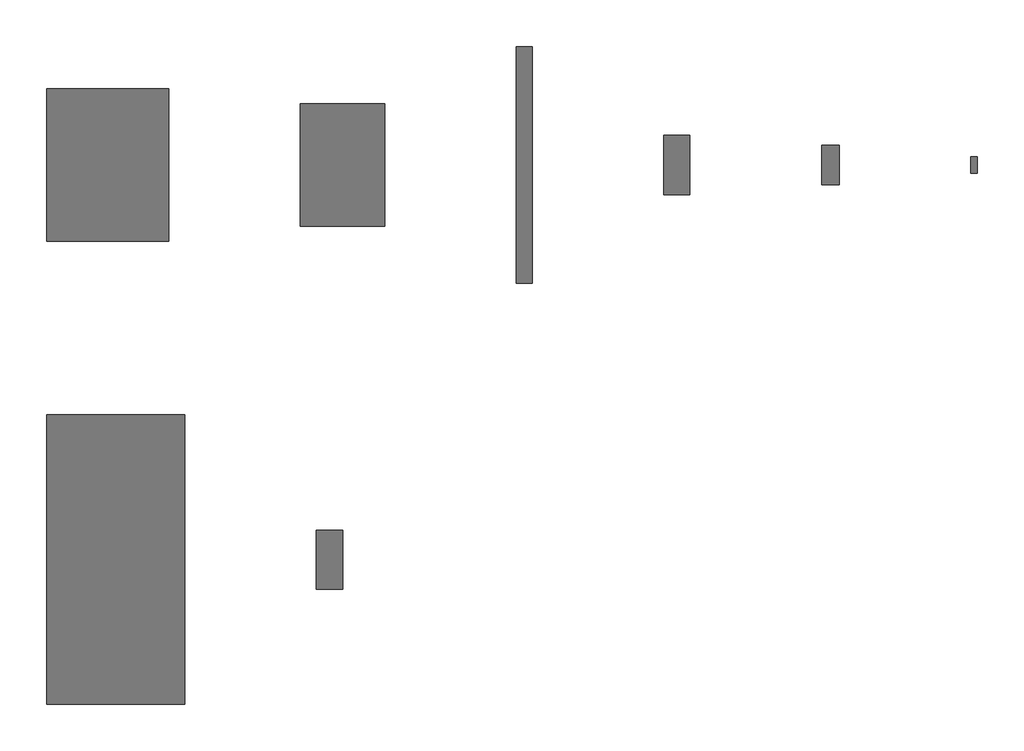
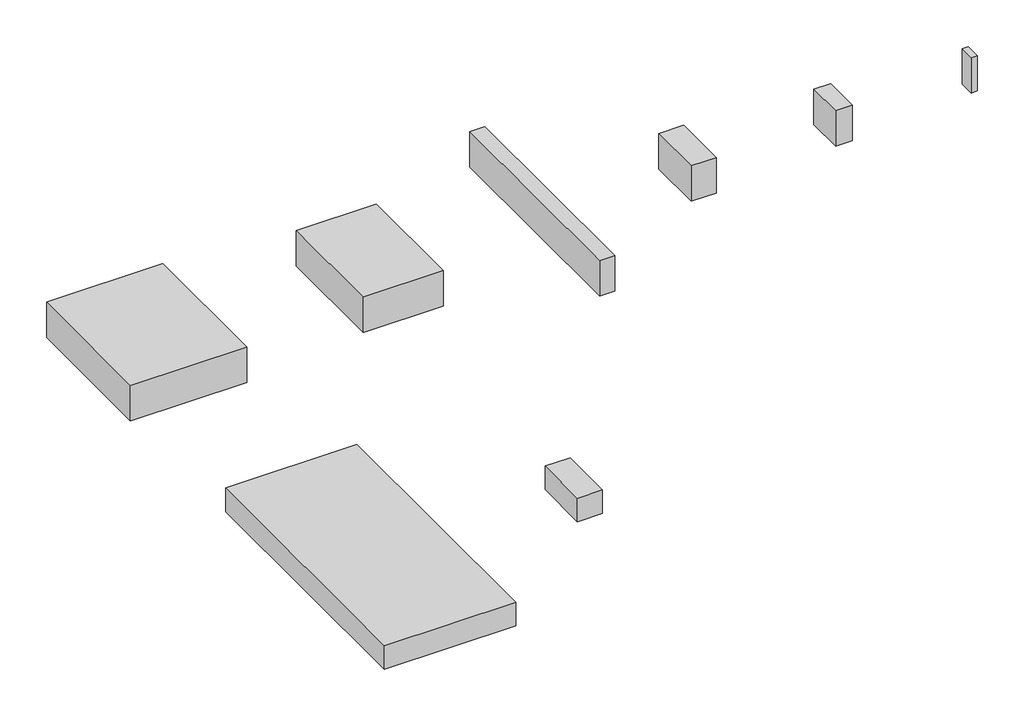
# One storey: 8 proxies.
"""IFC4 building model written with IfcOpenShell, lengths in millimetres."""

import ifcopenshell
import ifcopenshell.guid

model = None  # the IFC model being written
_history = None  # IfcOwnerHistory: only IFC2X3 demands one
_inside = {}  # id of a spatial element -> (the spatial element, [elements in it])
_under = {}  # id of a project, library or spatial element -> (it, [spatial elements below it])
_declared = {}  # id of a project -> (the project, [libraries it declares])
_typed = {}  # id of a type object -> (the type object, [elements of that type])
_made_of = {}  # id of a material, layer set ... -> (it, [elements and type objects made of it])


def new_model(schema):
    """Start an empty IFC model of exactly this schema.

    Asked for "IFC4X3", IfcOpenShell would pick the latest addendum, in which some entities
    have other attributes; the version numbers below select the first issue.
    IFC2X3 requires an IfcOwnerHistory on every rooted entity: one is made here for all.
    """
    global model, _history
    if schema == "IFC4X3":
        model = ifcopenshell.file(schema_version=(4, 3, 0, 0))
    else:
        model = ifcopenshell.file(schema=schema)
    _inside.clear()
    _under.clear()
    _declared.clear()
    _typed.clear()
    _made_of.clear()
    _history = None
    if model.schema == "IFC2X3":
        org = make("IfcOrganization", Name="unknown")
        user = make(
            "IfcPersonAndOrganization",
            ThePerson=make("IfcPerson", FamilyName="unknown"),
            TheOrganization=org,
        )
        app = make(
            "IfcApplication",
            ApplicationDeveloper=org,
            Version="unknown",
            ApplicationFullName="unknown",
            ApplicationIdentifier="unknown",
        )
        _history = make(
            "IfcOwnerHistory",
            OwningUser=user,
            OwningApplication=app,
            ChangeAction="ADDED",
            CreationDate=0,
        )
    return model


def make(cls, **values):
    """One entity of the class cls with the attributes given. An attribute that is None is left unset."""
    return model.create_entity(
        cls, **{name: value for name, value in values.items() if value is not None}
    )


def rooted(cls, **values):
    """An entity with a GlobalId (a new one), such as an element, a storey or a relation."""
    return make(cls, GlobalId=ifcopenshell.guid.new(), OwnerHistory=_history, **values)


def si_unit(unit_type, name, prefix=None):
    """IfcSIUnit, for example si_unit("LENGTHUNIT", "METRE", prefix="MILLI")."""
    return make("IfcSIUnit", UnitType=unit_type, Prefix=prefix, Name=name)


def assignment(units):
    """IfcUnitAssignment: the units of a project."""
    return None if units is None else make("IfcUnitAssignment", Units=units)


def point(xyz):
    """IfcCartesianPoint."""
    return None if xyz is None else make("IfcCartesianPoint", Coordinates=xyz)


def direction(xyz):
    """IfcDirection."""
    return None if xyz is None else make("IfcDirection", DirectionRatios=xyz)


def frame(location, z_axis=None, x_axis=None):
    """IfcAxis2Placement3D, a coordinate frame: its origin and axes. An axis left out is left unset."""
    return make(
        "IfcAxis2Placement3D",
        Location=point(location),
        Axis=direction(z_axis),
        RefDirection=direction(x_axis),
    )


def origin():
    """The frame at (0, 0, 0) with its axes left unset."""
    return frame((0.0, 0.0, 0.0))


def origin_with_axes():
    """The frame at (0, 0, 0) with the z axis (0, 0, 1) and the x axis (1, 0, 0) written out."""
    return frame((0.0, 0.0, 0.0), z_axis=(0.0, 0.0, 1.0), x_axis=(1.0, 0.0, 0.0))


def place(relative_to, where):
    """IfcLocalPlacement: puts the frame where relative to a parent placement (None: the world)."""
    return make(
        "IfcLocalPlacement", PlacementRelTo=relative_to, RelativePlacement=where
    )


def context(
    kind, dimensions, precision=None, world=None, true_north=None, identifier=None
):
    """IfcGeometricRepresentationContext, for example the 3D "Model" context."""
    return make(
        "IfcGeometricRepresentationContext",
        ContextIdentifier=identifier,
        ContextType=kind,
        CoordinateSpaceDimension=dimensions,
        Precision=precision,
        WorldCoordinateSystem=world,
        TrueNorth=true_north,
    )


def project(units=None, contexts=None):
    """IfcProject with its units and contexts."""
    return rooted(
        "IfcProject",
        Name="project",
        RepresentationContexts=contexts,
        UnitsInContext=assignment(units),
    )


def spatial(cls, under=None, at=None, **own):
    """A site, building, storey or space (cls), placed at a placement, below another one or the project."""
    s = rooted(cls, ObjectPlacement=at, **own)
    if under is not None:
        _under.setdefault(under.id(), (under, []))[1].append(s)
    return s


def polyline(points):
    """IfcPolyline through the points."""
    return make("IfcPolyline", Points=[point(p) for p in points])


def outline(outer, holes=None, kind="AREA"):
    """IfcArbitraryClosedProfileDef: a profile drawn as a closed curve; with holes, ...WithVoids."""
    if holes is None:
        return make("IfcArbitraryClosedProfileDef", ProfileType=kind, OuterCurve=outer)
    return make(
        "IfcArbitraryProfileDefWithVoids",
        ProfileType=kind,
        OuterCurve=outer,
        InnerCurves=holes,
    )


def extrude(swept, where, along, depth):
    """IfcExtrudedAreaSolid: the profile swept, set in the frame where, extruded along a direction by depth."""
    return make(
        "IfcExtrudedAreaSolid",
        SweptArea=swept,
        Position=where,
        ExtrudedDirection=direction(along),
        Depth=depth,
    )


def shape(context_of_items, identifier, shape_type, items):
    """IfcShapeRepresentation: the items that make up one representation, for example the "Body"."""
    return make(
        "IfcShapeRepresentation",
        ContextOfItems=context_of_items,
        RepresentationIdentifier=identifier,
        RepresentationType=shape_type,
        Items=items,
    )


def source(mapping_origin, context_of_items, identifier, shape_type, items):
    """IfcRepresentationMap: a shape defined once, which mapped items show again and again."""
    return make(
        "IfcRepresentationMap",
        MappingOrigin=mapping_origin,
        MappedRepresentation=shape(context_of_items, identifier, shape_type, items),
    )


def transform(
    local_origin,
    x_axis=None,
    y_axis=None,
    z_axis=None,
    scale=None,
    scale2=None,
    scale3=None,
    uniform=True,
):
    """IfcCartesianTransformationOperator3D, or its non-uniform kind. x_axis, y_axis, z_axis: its Axis1, 2, 3."""
    if uniform:
        return make(
            "IfcCartesianTransformationOperator3D",
            Axis1=direction(x_axis),
            Axis2=direction(y_axis),
            LocalOrigin=point(local_origin),
            Scale=scale,
            Axis3=direction(z_axis),
        )
    return make(
        "IfcCartesianTransformationOperator3DnonUniform",
        Axis1=direction(x_axis),
        Axis2=direction(y_axis),
        LocalOrigin=point(local_origin),
        Scale=scale,
        Axis3=direction(z_axis),
        Scale2=scale2,
        Scale3=scale3,
    )


def mapped(mapping_source, mapping_target):
    """IfcMappedItem: shows the shape of a source again, moved by a transform."""
    return make(
        "IfcMappedItem", MappingSource=mapping_source, MappingTarget=mapping_target
    )


def made_of(thing, what):
    """Note that an element or type object is made of a material, layer set ...; save() writes the relation."""
    if what is not None:
        _made_of.setdefault(what.id(), (what, []))[1].append(thing)
    return thing


def element(
    cls,
    number,
    at=None,
    inside=None,
    cuts=None,
    type_object=None,
    material=None,
    context=None,
    identifier="Body",
    shape_type=None,
    held_by="IfcProductDefinitionShape",
    body=None,
    shapes=None,
    **own,
):
    """One element of the class cls, such as IfcWall. Its Tag is "e" and its number.

    at: its placement. inside: the storey or other place that contains it. cuts: it is an
    opening in that element (IfcRelVoidsElement). A single representation is given by context,
    identifier, shape_type and body (its items); several are given by shapes. held_by: the class
    of the entity that holds the representations. save() writes the other relations.
    """
    e = rooted(cls, Tag="e%d" % number, ObjectPlacement=at, **own)
    if body is not None:
        shapes = [shape(context, identifier, shape_type, body)]
    if shapes is not None:
        e.Representation = make(held_by, Representations=shapes)
    if inside is not None:
        _inside.setdefault(inside.id(), (inside, []))[1].append(e)
    if cuts is not None:
        rooted(
            "IfcRelVoidsElement", RelatingBuildingElement=cuts, RelatedOpeningElement=e
        )
    if type_object is not None:
        _typed.setdefault(type_object.id(), (type_object, []))[1].append(e)
    return made_of(e, material)


def aggregate(whole, parts):
    """IfcRelAggregates: a whole, such as a stair, and the parts it consists of."""
    return rooted("IfcRelAggregates", RelatingObject=whole, RelatedObjects=parts)


def save(model, path):
    """Write the relations noted so far, then the file.

    IfcRelAggregates (storeys below a building ...), IfcRelContainedInSpatialStructure (elements
    in a storey), IfcRelDefinesByType, IfcRelAssociatesMaterial and IfcRelDeclares: one each for
    every whole, place, type object, material and project.
    """
    for whole, parts in _under.values():
        aggregate(whole, parts)
    for where, things in _inside.values():
        rooted(
            "IfcRelContainedInSpatialStructure",
            RelatedElements=things,
            RelatingStructure=where,
        )
    for kind, things in _typed.values():
        rooted("IfcRelDefinesByType", RelatedObjects=things, RelatingType=kind)
    for what, things in _made_of.values():
        rooted("IfcRelAssociatesMaterial", RelatedObjects=things, RelatingMaterial=what)
    for by, libraries in _declared.values():
        rooted("IfcRelDeclares", RelatingContext=by, RelatedDefinitions=libraries)
    model.write(path)


def generic_models_29bcd6f9(model_context):
    return source(origin(), model_context, "Body", "SweptSolid", [
        extrude(outline(polyline([(2000.0, 4500.0), (2000.0, -4500.0), (-2000.0, -4500.0), (-2000.0, 4500.0), (2000.0, 4500.0)])), origin_with_axes(), (0.0, 0.0, 1.0), 6000.0),
    ])


def generic_models_a454a2aa(model_context):
    return source(origin(), model_context, "Body", "SweptSolid", [
        extrude(outline(polyline([(10500.0, 22000.0), (10500.0, -22000.0), (-10500.0, -22000.0), (-10500.0, 22000.0), (10500.0, 22000.0)])), origin_with_axes(), (0.0, 0.0, 1.0), 4000.0),
    ])


def generic_models_73802227(model_context):
    return source(origin(), model_context, "Body", "SweptSolid", [
        extrude(outline(polyline([(2000.0, 4500.0), (2000.0, -4500.0), (-2000.0, -4500.0), (-2000.0, 4500.0), (2000.0, 4500.0)])), origin_with_axes(), (0.0, 0.0, 1.0), 4000.0),
    ])


def generic_models_d82b1902(model_context):
    return source(origin(), model_context, "Body", "SweptSolid", [
        extrude(outline(polyline([(9300.0, 11600.0), (9300.0, -11600.0), (-9300.0, -11600.0), (-9300.0, 11600.0), (9300.0, 11600.0)])), origin_with_axes(), (0.0, 0.0, 1.0), 6000.0),
    ])


def generic_models_21711933(model_context):
    return source(origin(), model_context, "Body", "SweptSolid", [
        extrude(outline(polyline([(6400.0, 9300.0), (6400.0, -9300.0), (-6400.0, -9300.0), (-6400.0, 9300.0), (6400.0, 9300.0)])), origin_with_axes(), (0.0, 0.0, 1.0), 6000.0),
    ])


def generic_models_03d31222(model_context):
    return source(origin(), model_context, "Body", "SweptSolid", [
        extrude(outline(polyline([(1200.0, 18000.0), (1200.0, -18000.0), (-1200.0, -18000.0), (-1200.0, 18000.0), (1200.0, 18000.0)])), origin_with_axes(), (0.0, 0.0, 1.0), 6000.0),
    ])


def generic_models_5634f436(model_context):
    return source(origin(), model_context, "Body", "SweptSolid", [
        extrude(outline(polyline([(1350.0, 3000.0), (1350.0, -3000.0), (-1350.0, -3000.0), (-1350.0, 3000.0), (1350.0, 3000.0)])), origin_with_axes(), (0.0, 0.0, 1.0), 6000.0),
    ])


def generic_models_71e2440f(model_context):
    return source(origin(), model_context, "Body", "SweptSolid", [
        extrude(outline(polyline([(500.0, 1250.0), (500.0, -1250.0), (-500.0, -1250.0), (-500.0, 1250.0), (500.0, 1250.0)])), origin_with_axes(), (0.0, 0.0, 1.0), 6000.0),
    ])


model = new_model("IFC4")

# Units and contexts
model_context = context("Model", 3, world=origin())
ifc_project = project(units=[si_unit("LENGTHUNIT", "METRE", prefix="MILLI")], contexts=[model_context])

# Site, building, storey
site = spatial("IfcSite", under=ifc_project)
building = spatial("IfcBuilding", under=site)
storey = spatial("IfcBuildingStorey", under=building, Name="T.O.C(H.P)", Elevation=4050.0)

# Proxies
placement = place(None, origin())
generic_models_shape = generic_models_29bcd6f9(model_context)
element("IfcBuildingElementProxy", 1, Name="Space Planning Box_hec : Space Planning Box_hec", ObjectType="Space Planning Box_hec : Space Planning Box_hec", at=placement, inside=storey, context=model_context, shape_type="MappedRepresentation", body=[
    mapped(generic_models_shape, transform((95800.0, 114000.0, 4050.0), x_axis=(1.0, 0.0, 0.0), y_axis=(0.0, 1.0, 0.0), z_axis=(0.0, 0.0, 1.0))),
])
generic_models_2_shape = generic_models_a454a2aa(model_context)
element("IfcBuildingElementProxy", 2, Name="Space Planning Box_hec : Space Planning Box_hec", ObjectType="Space Planning Box_hec : Space Planning Box_hec", at=placement, inside=storey, context=model_context, shape_type="MappedRepresentation", body=[
    mapped(generic_models_2_shape, transform((10500.0, 54000.0, 4650.0), x_axis=(1.0, 0.0, 0.0), y_axis=(0.0, 1.0, 0.0), z_axis=(0.0, 0.0, 1.0))),
])
generic_models_3_shape = generic_models_73802227(model_context)
element("IfcBuildingElementProxy", 3, Name="Space Planning Box_hec : Space Planning Box_hec", ObjectType="Space Planning Box_hec : Space Planning Box_hec", at=placement, inside=storey, context=model_context, shape_type="MappedRepresentation", body=[
    mapped(generic_models_3_shape, transform((43000.0, 54000.0, 4650.0), x_axis=(1.0, 0.0, 0.0), y_axis=(0.0, 1.0, 0.0), z_axis=(0.0, 0.0, 1.0))),
])
generic_models_4_shape = generic_models_d82b1902(model_context)
element("IfcBuildingElementProxy", 4, Name="Space Planning Box_hec : Space Planning Box_hec", ObjectType="Space Planning Box_hec : Space Planning Box_hec", at=placement, inside=storey, context=model_context, shape_type="MappedRepresentation", body=[
    mapped(generic_models_4_shape, transform((9300.0, 114000.0, 4050.0), x_axis=(1.0, 0.0, 0.0), y_axis=(0.0, 1.0, 0.0), z_axis=(0.0, 0.0, 1.0))),
])
generic_models_5_shape = generic_models_21711933(model_context)
element("IfcBuildingElementProxy", 5, Name="Space Planning Box_hec : Space Planning Box_hec", ObjectType="Space Planning Box_hec : Space Planning Box_hec", at=placement, inside=storey, context=model_context, shape_type="MappedRepresentation", body=[
    mapped(generic_models_5_shape, transform((45000.0, 114000.0, 4050.0), x_axis=(1.0, 0.0, 0.0), y_axis=(0.0, 1.0, 0.0), z_axis=(0.0, 0.0, 1.0))),
])
generic_models_6_shape = generic_models_03d31222(model_context)
element("IfcBuildingElementProxy", 6, Name="Space Planning Box_hec : Space Planning Box_hec", ObjectType="Space Planning Box_hec : Space Planning Box_hec", at=placement, inside=storey, context=model_context, shape_type="MappedRepresentation", body=[
    mapped(generic_models_6_shape, transform((72600.0, 114000.0, 4050.0), x_axis=(1.0, 0.0, 0.0), y_axis=(0.0, 1.0, 0.0), z_axis=(0.0, 0.0, 1.0))),
])
generic_models_7_shape = generic_models_5634f436(model_context)
element("IfcBuildingElementProxy", 7, Name="Space Planning Box_hec : Space Planning Box_hec", ObjectType="Space Planning Box_hec : Space Planning Box_hec", at=placement, inside=storey, context=model_context, shape_type="MappedRepresentation", body=[
    mapped(generic_models_7_shape, transform((119150.0, 114000.0, 4050.0), x_axis=(1.0, 0.0, 0.0), y_axis=(0.0, 1.0, 0.0), z_axis=(0.0, 0.0, 1.0))),
])
generic_models_8_shape = generic_models_71e2440f(model_context)
element("IfcBuildingElementProxy", 8, Name="Space Planning Box_hec : Space Planning Box_hec", ObjectType="Space Planning Box_hec : Space Planning Box_hec", at=placement, inside=storey, context=model_context, shape_type="MappedRepresentation", body=[
    mapped(generic_models_8_shape, transform((141000.0, 114000.0, 4050.0), x_axis=(1.0, 0.0, 0.0), y_axis=(0.0, 1.0, 0.0), z_axis=(0.0, 0.0, 1.0))),
])

save(model, "model.ifc")

# Revit data of these elements
# Type "Space Planning Box_hec : Space Planning Box_hec"
#   Type Comments = "..."
#   Room Name [instance default] = "?"
#   Interior Finish [instance default] = ""
#   Exterior Finish [instance default] = ""
#   Department [instance default] = ""
#   Assembly Code = "..."
#   Width [instance default] = 1524 mm
#   Program Area [instance default] = 0.00 m²
#   Length [instance default] = 1524 mm
#   Height [instance default] = 1524 mm
#   Area [instance default] = 2.32258 m²
#   Fill Color [instance default] = Cyan
#   Default Elevation = 0
# Element 1 (IfcBuildingElementProxy, "Space Planning Box_hec : Space Planning Box_hec")
#   Room Name = "Stairway"
#   Interior Finish = "IF2"
#   Exterior Finish = "EF1"
#   Department = "AR"
#   Width = 4000 mm
#   Program Area = 36.00 m²
#   Length = 9000 mm
#   Height = 6000 mm
#   Area = 36.00 m²
#   Fill Color = Cyan
#   Phase Created = New Construction
#   Materials on its faces: "Cyan"
# Element 2 (IfcBuildingElementProxy, "Space Planning Box_hec : Space Planning Box_hec")
#   Room Name = "Cable Room"
#   Interior Finish = "IF1"
#   Exterior Finish = "EF1"
#   Department = "EL"
#   Width = 21000 mm
#   Program Area = 924.00 m²
#   Length = 44000 mm
#   Height = 4000 mm
#   Area = 924.00 m²
#   Fill Color = Cyan
#   Phase Created = New Construction
#   Materials on its faces: "Cyan"
# Element 3 (IfcBuildingElementProxy, "Space Planning Box_hec : Space Planning Box_hec")
#   Room Name = "Stairway"
#   Interior Finish = "IF2"
#   Exterior Finish = "EF1"
#   Department = "EL"
#   Width = 4000 mm
#   Program Area = 36.00 m²
#   Length = 9000 mm
#   Height = 4000 mm
#   Area = 36.00 m²
#   Fill Color = Cyan
#   Phase Created = New Construction
#   Materials on its faces: "Cyan"
# Element 4 (IfcBuildingElementProxy, "Space Planning Box_hec : Space Planning Box_hec")
#   Room Name = "Electronic Room"
#   Interior Finish = "IF1"
#   Exterior Finish = "EF1"
#   Department = "CI"
#   Width = 18600 mm
#   Program Area = 431.52 m²
#   Length = 23200 mm
#   Height = 6000 mm
#   Area = 431.52 m²
#   Fill Color = Cyan
#   Phase Created = New Construction
#   Materials on its faces: "Cyan"
# Element 5 (IfcBuildingElementProxy, "Space Planning Box_hec : Space Planning Box_hec")
#   Room Name = "Electrical Room"
#   Interior Finish = "IF1"
#   Exterior Finish = "EF1"
#   Department = "EL"
#   Width = 12800 mm
#   Program Area = 238.08 m²
#   Length = 18600 mm
#   Height = 6000 mm
#   Area = 238.08 m²
#   Fill Color = Cyan
#   Phase Created = New Construction
#   Materials on its faces: "Cyan"
# Element 6 (IfcBuildingElementProxy, "Space Planning Box_hec : Space Planning Box_hec")
#   Room Name = "Corridor"
#   Interior Finish = "IF2-1"
#   Exterior Finish = "EF1"
#   Department = "AR"
#   Width = 2400 mm
#   Program Area = 86.40 m²
#   Length = 36000 mm
#   Height = 6000 mm
#   Area = 86.40 m²
#   Fill Color = Cyan
#   Phase Created = New Construction
#   Materials on its faces: "Cyan"
# Element 7 (IfcBuildingElementProxy, "Space Planning Box_hec : Space Planning Box_hec")
#   Room Name = "Duct Shaft"
#   Interior Finish = "NA"
#   Exterior Finish = "EF1"
#   Department = "HV"
#   Width = 2700 mm
#   Program Area = 16.20 m²
#   Length = 6000 mm
#   Height = 6000 mm
#   Area = 16.20 m²
#   Fill Color = Cyan
#   Phase Created = New Construction
#   Materials on its faces: "Cyan"
# Element 8 (IfcBuildingElementProxy, "Space Planning Box_hec : Space Planning Box_hec")
#   Room Name = "Pipe Shaft"
#   Interior Finish = "NA"
#   Exterior Finish = "EF1"
#   Department = "HV"
#   Width = 1000 mm
#   Program Area = 2.50 m²
#   Length = 2500 mm
#   Height = 6000 mm
#   Area = 2.50 m²
#   Fill Color = Cyan
#   Phase Created = New Construction
#   Materials on its faces: "Cyan"
# Materials
#   "Cyan": class "Generic", colour RGB 0 255 255, transparency 0.2, Cost = 0
